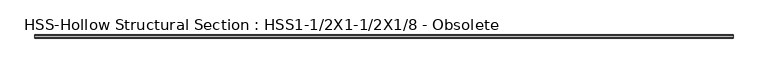
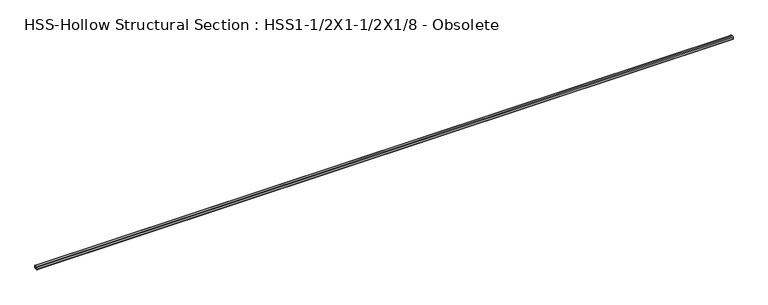
"""IFC4 building model written with IfcOpenShell, lengths in millimetres: beam geometry, HSS-Hollow Structural Section : HSS1-1/2X1-1/2X1/8 - Obsolete."""

from ifc_helpers import new_model, si_unit, point, frame, frame_2d, origin, place, context, project, spatial, polyline, circle_curve, trimmed, segment, composite_curve, outline, extrude, source, transform, mapped, element, save


def hss_hollow_structural_section_hss1_1_2x1_1_2x1_8_obsolete_c3719d16(model_context):
    return source(origin(), model_context, "Body", "SweptSolid", [
        extrude(outline(composite_curve([segment(polyline([(19.05, 13.1572), (19.05, -13.1572)]), True, "CONTINUOUS"), segment(trimmed(circle_curve(frame_2d((13.1572, -13.1572)), 5.8928), [point((19.05, -13.1572))], [point((13.1572, -19.05))], False, "CARTESIAN"), True, "CONTINUOUS"), segment(polyline([(13.1572, -19.05), (-13.1572, -19.05)]), True, "CONTINUOUS"), segment(trimmed(circle_curve(frame_2d((-13.1572, -13.1572)), 5.8928), [point((-13.1572, -19.05))], [point((-19.05, -13.1572))], False, "CARTESIAN"), True, "CONTINUOUS"), segment(polyline([(-19.05, -13.1572), (-19.05, 13.1572)]), True, "CONTINUOUS"), segment(trimmed(circle_curve(frame_2d((-13.1572, 13.1572)), 5.8928), [point((-19.05, 13.1572))], [point((-13.1572, 19.05))], False, "CARTESIAN"), True, "CONTINUOUS"), segment(polyline([(-13.1572, 19.05), (13.1572, 19.05)]), True, "CONTINUOUS"), segment(trimmed(circle_curve(frame_2d((13.1572, 13.1572)), 5.8928), [point((13.1572, 19.05))], [point((19.05, 13.1572))], False, "CARTESIAN"), True, "CONTINUOUS")], self_intersect=False), holes=[composite_curve([segment(trimmed(circle_curve(frame_2d((-13.1572, 13.1572)), 2.9464), [point((-13.1572, 16.1036))], [point((-16.1036, 13.1572))], True, "CARTESIAN"), True, "CONTINUOUS"), segment(polyline([(-16.1036, 13.1572), (-16.1036, -13.1572)]), True, "CONTINUOUS"), segment(trimmed(circle_curve(frame_2d((-13.1572, -13.1572)), 2.9464), [point((-16.1036, -13.1572))], [point((-13.1572, -16.1036))], True, "CARTESIAN"), True, "CONTINUOUS"), segment(polyline([(-13.1572, -16.1036), (13.1572, -16.1036)]), True, "CONTINUOUS"), segment(trimmed(circle_curve(frame_2d((13.1572, -13.1572)), 2.9464), [point((13.1572, -16.1036))], [point((16.1036, -13.1572))], True, "CARTESIAN"), True, "CONTINUOUS"), segment(polyline([(16.1036, -13.1572), (16.1036, 13.1572)]), True, "CONTINUOUS"), segment(trimmed(circle_curve(frame_2d((13.1572, 13.1572)), 2.9464), [point((16.1036, 13.1572))], [point((13.1572, 16.1036))], True, "CARTESIAN"), True, "CONTINUOUS"), segment(polyline([(13.1572, 16.1036), (-13.1572, 16.1036)]), True, "CONTINUOUS")], self_intersect=False)]), frame((-4286.2500001, 0.0, 0.0), z_axis=(1.0, 0.0, 0.0), x_axis=(0.0, 1.0, 0.0)), (0.0, 0.0, 1.0), 8572.5000002),
    ])


if __name__ == "__main__":
    model = new_model("IFC4")
    model_context = context("Model", 3, world=origin())
    ifc_project = project(units=[si_unit("LENGTHUNIT", "METRE", prefix="MILLI")], contexts=[model_context])
    site = spatial("IfcSite", under=ifc_project)
    building = spatial("IfcBuilding", under=site)
    placement = place(None, origin())
    hss_hollow_structural_section_hss1_1_2x1_1_2x1_8_obsolete_shape = hss_hollow_structural_section_hss1_1_2x1_1_2x1_8_obsolete_c3719d16(model_context)
    element("IfcBeam", 1, ObjectType="HSS-Hollow Structural Section : HSS1-1/2X1-1/2X1/8 - Obsolete", at=placement, inside=building, context=model_context, shape_type="MappedRepresentation", body=[
        mapped(hss_hollow_structural_section_hss1_1_2x1_1_2x1_8_obsolete_shape, transform((0.0, 0.0, 0.0), x_axis=(1.0, 0.0, 0.0), y_axis=(0.0, 1.0, 0.0), z_axis=(0.0, 0.0, 1.0))),
    ])
    save(model, "model.ifc")

# Revit data of these elements
# Type "HSS-Hollow Structural Section : HSS1-1/2X1-1/2X1/8 - Obsolete"
#   Assembly Code = "B10"
#   Shape = "Square"
#   W = 2.19
#   Ht = 0' - 1 1/2"
#   Length [instance default] = 5' - 0"
#   b = 0' - 1 1/2"
#   kr = 0' - 0.232"
#   t = 0' - 0.116"
#   A = 0.00423611 SF
#   Structural Material [instance default] = 1 1/2" X 1 1/2" x 1/8" ALUM. TUBE
# Element 1 (IfcBeam, "HSS-Hollow Structural Section : HSS1-1/2X1-1/2X1/8 - Obsolete")
#   Materials on its faces: "1 1/2\" X 1 1/2\" x 1/8\" ALUM. TUBE"
# Materials
#   "1 1/2\" X 1 1/2\" x 1/8\" ALUM. TUBE": class "Metal", colour RGB 199 199 199, transparency 0, Description = "Carbon steel", Cost = 0
